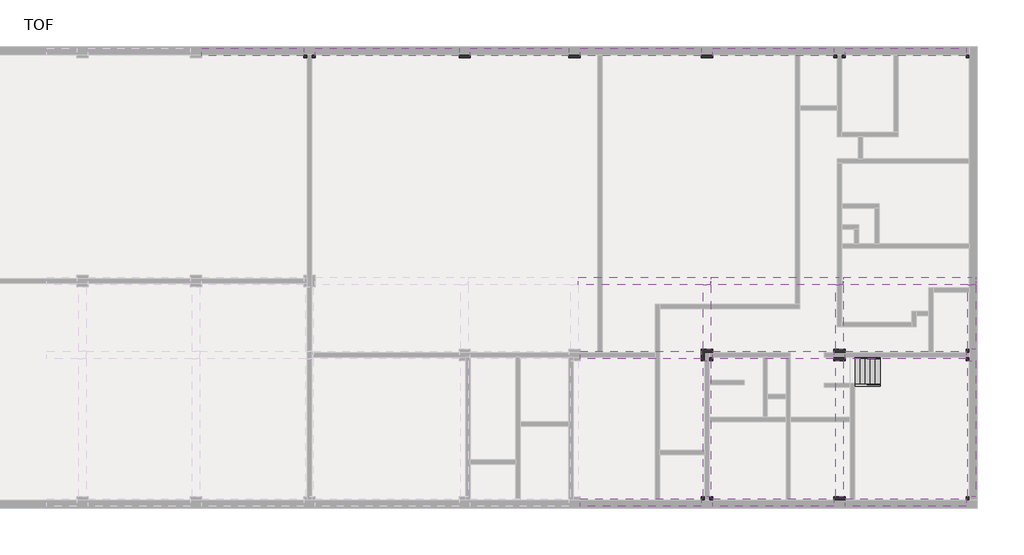
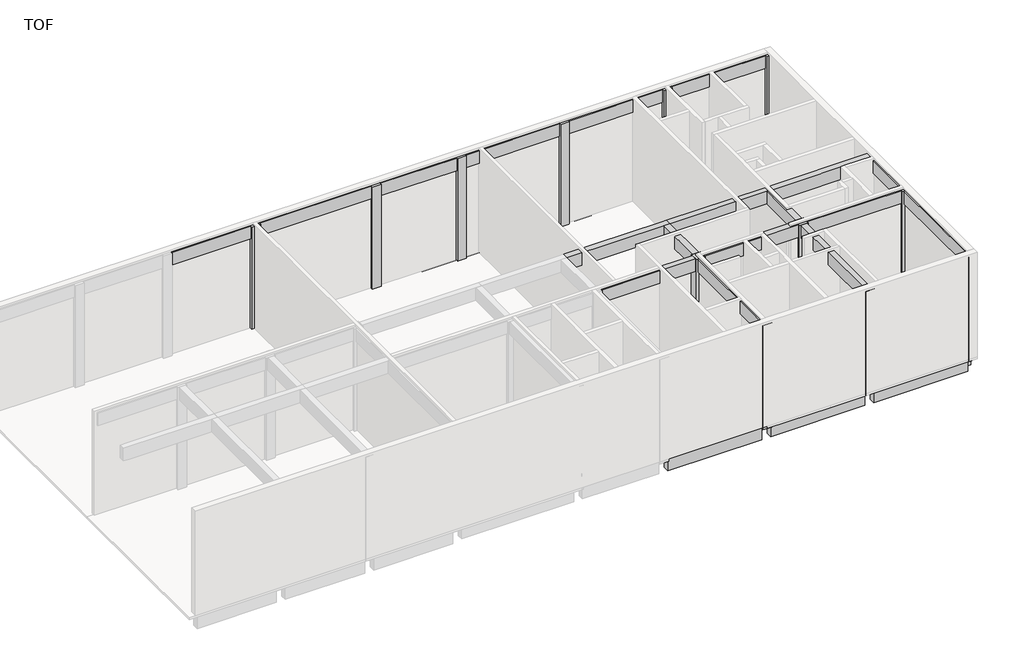
# One storey, part 3 of 3: 32 beams, 12 columns, 2 members, 2 railings, 1 stair flight.
# Revit data of these elements (continued)
# Type "RC Beam_Rectangular : H_SB_ACB_B400xH900"
#   중앙부 하부근 = ""
#   중앙부 상부근 = ""
#   중앙부 보조근 = ""
#   중앙부 늑근 = ""
#   외단부 하부근 = ""
#   외단부 상부근 = ""
#   외단부 보조근 = ""
#   외단부 늑근 = ""
#   부호 = "TG3"
#   내단부 하부근 = ""
#   내단부 상부근 = ""
#   내단부 보조근 = ""
#   내단부 늑근 = ""
#   ALL 하부근 = "3-D20"
#   ALL 상부근 = "3-D20"
#   ALL 보조근 = ""
#   ALL 늑근 = "2-D10 @120"
#   Width = 400.000 mm
#   Height = 900.000 mm
#   Length [instance default] = 1524.000 mm
#   b = 400.000 mm
#   h = 900.000 mm
#   hec_material3 [instance default] = none
#   hec_material2 [instance default] = none
#   hec_material1 [instance default] = none
#   Structural Material [instance default] = none
#   Assembly Code = ""
# Type "RC_Column_Rectangular : H_SC_ACC_W600xL600"
#   Width = 600.000 mm
#   Length = 600.000 mm
#   hec_material3 [instance default] = none
#   hec_material2 [instance default] = none
#   hec_material1 [instance default] = none
#   Structural Material [instance default] = none
#   Description = (empty or 0)
# Type "H_RL_AMH_Steel Handrail_H1100"
#   built-in parameter 1008619 = -0.082021 (stored number, unit not read)
#   built-in parameter 1008612 = 0.019685 (stored number, unit not read)
#   built-in parameter 1008611 = 0.019685 (stored number, unit not read)
#   built-in parameter 1008609 = 0.902231 (stored number, unit not read)
#   built-in parameter 1008604 = 0.19685 (stored number, unit not read)
#   built-in parameter 1008603 = 0.164042 (stored number, unit not read)
#   Railing Height = 1100.000 mm
#   built-in parameter 1008630 = 2
#   built-in parameter 1008610 = 1
# Elements 1, 2, 3, 4, 5, 6, 7, 8, 9, 10, 11, 12, 13, 14, 15, 16, 17, 18, 19, 20, 21, 22, 23, 24, 25, 26, 27, 28, 29, 30, 31, 32 (IfcBeam, "RC Beam_Rectangular : H_SB_ACB_B400xH900")
#   hec_material3 = none
#   hec_material2 = none
#   hec_material1 = none
#   Structural Material = none
#   Phase Created = New Construction
# Elements 33, 34, 35, 36, 37, 38, 39, 40, 41, 42, 43, 44 (IfcColumn, "RC_Column_Rectangular : H_SC_ACC_W600xL600")
#   Comments = ""
#   hec_material3 = none
#   hec_material2 = none
#   hec_material1 = none
#   Structural Material = none
#   Phase Created = New Construction
# Element 45 (IfcMember, "Stringer - 75 mm Width 2")
#   Phase Created = New Construction
# Element 46 (IfcMember, "Stringer - Channel 75 mm Width")
#   Phase Created = New Construction
# Elements 47, 48 (IfcRailing, "H_RL_AMH_Steel Handrail_H1100")
#   Phase Created = New Construction
# Element 49 (IfcStairFlight, "철골계단")
#   Phase Created = New Construction
